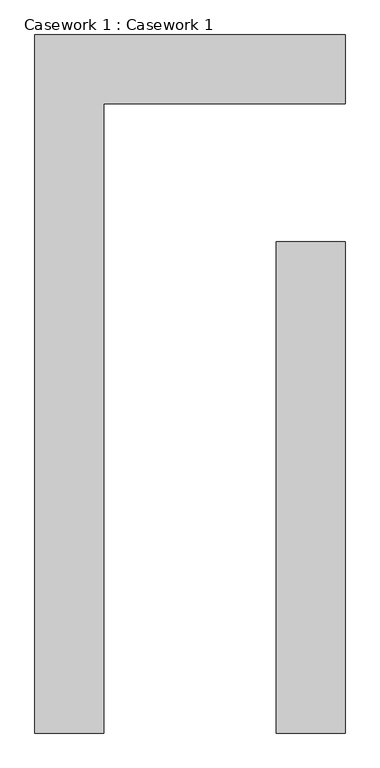
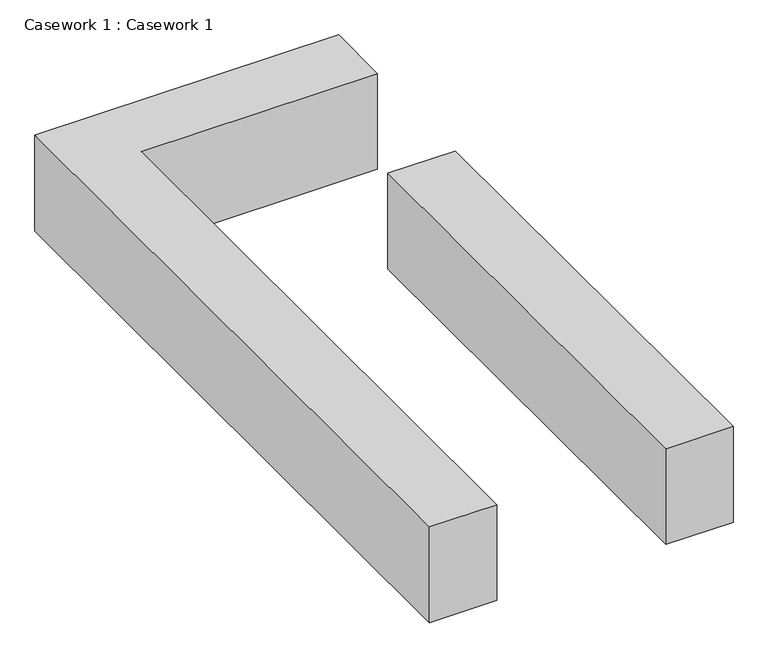
"""IFC4 building model written with IfcOpenShell, lengths in millimetres: furniture geometry, Casework 1 : Casework 1."""

from ifc_helpers import new_model, si_unit, origin, origin_with_axes, place, context, project, spatial, polyline, outline, extrude, source, transform, mapped, element, save


def casework_1_casework_1_6d664a8f(model_context):
    return source(origin(), model_context, "Body", "SweptSolid", [
        extrude(outline(polyline([(653450.3117239, -573802.8195091), (653450.3117239, -567627.8413841), (656193.5117239, -567627.8413841), (656193.5117239, -568237.4413841), (654059.9117239, -568237.4413841), (654059.9117239, -573802.8195091), (653450.3117239, -573802.8195091)])), origin_with_axes(), (0.0, 0.0, 1.0), 914.4),
        extrude(outline(polyline([(655583.9117239, -573802.8195091), (655583.9117239, -569456.6413841), (656193.5117239, -569456.6413841), (656193.5117239, -573802.8195091), (655583.9117239, -573802.8195091)])), origin_with_axes(), (0.0, 0.0, 1.0), 914.4),
    ])


if __name__ == "__main__":
    model = new_model("IFC4")
    model_context = context("Model", 3, world=origin())
    ifc_project = project(units=[si_unit("LENGTHUNIT", "METRE", prefix="MILLI")], contexts=[model_context])
    site = spatial("IfcSite", under=ifc_project)
    building = spatial("IfcBuilding", under=site)
    placement = place(None, origin())
    casework_1_casework_1_shape = casework_1_casework_1_6d664a8f(model_context)
    element("IfcFurniture", 1, ObjectType="Casework 1 : Casework 1", at=placement, inside=building, context=model_context, shape_type="MappedRepresentation", body=[
        mapped(casework_1_casework_1_shape, transform((0.0, 0.0, 0.0), x_axis=(1.0, 0.0, 0.0), y_axis=(0.0, 1.0, 0.0), z_axis=(0.0, 0.0, 1.0))),
    ])
    save(model, "model.ifc")
